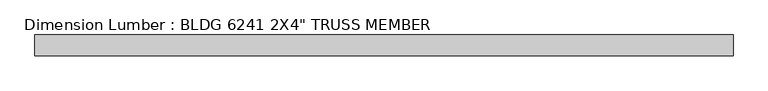
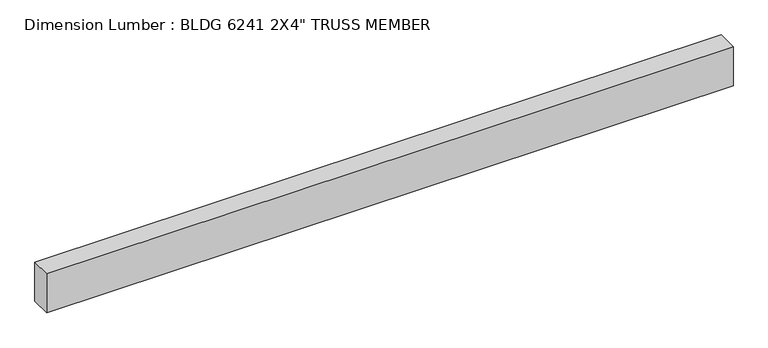
"""IFC4 building model written with IfcOpenShell, lengths in millimetres: beam geometry."""

from ifc_helpers import new_model, si_unit, frame, origin, place, context, project, spatial, polyline, outline, extrude, source, transform, mapped, element, save


def beam_3de093d9(model_context):
    return source(origin(), model_context, "Body", "SweptSolid", [
        extrude(outline(polyline([(233.4866591, -25.4), (-1464.867127, -25.4), (-1464.867127, 25.4), (233.4866591, 25.4), (233.4866591, -25.4)])), frame((0.0, 0.0, -50.8), z_axis=(0.0, 0.0, 1.0), x_axis=(1.0, 0.0, 0.0)), (0.0, 0.0, 1.0), 101.6),
    ])


if __name__ == "__main__":
    model = new_model("IFC4")
    model_context = context("Model", 3, world=origin())
    ifc_project = project(units=[si_unit("LENGTHUNIT", "METRE", prefix="MILLI")], contexts=[model_context])
    site = spatial("IfcSite", under=ifc_project)
    building = spatial("IfcBuilding", under=site)
    placement = place(None, origin())
    beam_shape = beam_3de093d9(model_context)
    element("IfcBeam", 1, ObjectType="Dimension Lumber : BLDG 6241 2X4\" TRUSS MEMBER", at=placement, inside=building, context=model_context, shape_type="MappedRepresentation", body=[
        mapped(beam_shape, transform((0.0, 0.0, 0.0), x_axis=(1.0, 0.0, 0.0), y_axis=(0.0, 1.0, 0.0), z_axis=(0.0, 0.0, 1.0))),
    ])
    save(model, "model.ifc")

# Revit data of these elements
# Type "Dimension Lumber : BLDG 6241 2X4\" TRUSS MEMBER"
#   Assembly Code = "B10"
#   A = 0.273472 SF
#   Length [instance default] = 5' - 0"
#   b = 0' - 2"
#   d = 0' - 4"
#   Structural Material [instance default] = Softwood, Lumber
# Element 1 (IfcBeam, "Dimension Lumber : BLDG 6241 2X4\" TRUSS MEMBER")
#   Materials on its faces: "Softwood, Lumber"
# Materials
#   "Softwood, Lumber": class "Wood", colour RGB 223 192 134, transparency 0, Description = "Pinus Echinata", Cost = 0
